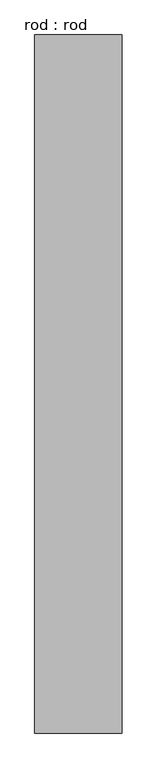
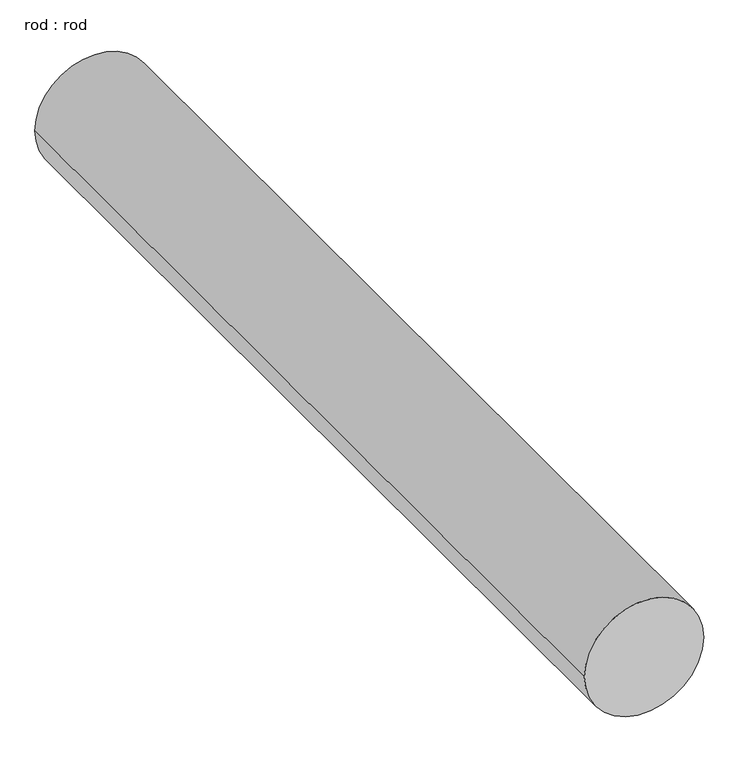
"""IFC4 building model written with IfcOpenShell, lengths in millimetres: proxy geometry, rod : rod."""

from ifc_helpers import new_model, si_unit, point, frame, frame_2d, origin, place, context, project, spatial, circle_curve, trimmed, segment, composite_curve, outline, extrude, source, transform, mapped, element, save


def rod_rod_74fe4f4c(model_context):
    return source(origin(), model_context, "Body", "SweptSolid", [
        extrude(outline(composite_curve([segment(trimmed(circle_curve(frame_2d((0.0108462, 0.0)), 200.0), [point((0.0108462, 200.0))], [point((0.0108462, -200.0))], False, "CARTESIAN"), True, "CONTINUOUS"), segment(trimmed(circle_curve(frame_2d((0.0108462, 0.0)), 200.0), [point((0.0108462, -200.0))], [point((0.0108462, 200.0))], False, "CARTESIAN"), True, "CONTINUOUS")], self_intersect=False)), frame((0.0, 2496.3000439, 0.0), z_axis=(0.0, 1.0, 0.0), x_axis=(0.0, 0.0, 1.0)), (0.0, 0.0, 1.0), 3192.8571429),
    ])


if __name__ == "__main__":
    model = new_model("IFC4")
    model_context = context("Model", 3, world=origin())
    ifc_project = project(units=[si_unit("LENGTHUNIT", "METRE", prefix="MILLI")], contexts=[model_context])
    site = spatial("IfcSite", under=ifc_project)
    building = spatial("IfcBuilding", under=site)
    placement = place(None, origin())
    rod_rod_shape = rod_rod_74fe4f4c(model_context)
    element("IfcBuildingElementProxy", 1, Name="rod : rod", ObjectType="rod : rod", at=placement, inside=building, context=model_context, shape_type="MappedRepresentation", body=[
        mapped(rod_rod_shape, transform((0.0, 0.0, 0.0), x_axis=(1.0, 0.0, 0.0), y_axis=(0.0, 1.0, 0.0), z_axis=(0.0, 0.0, 1.0))),
    ])
    save(model, "model.ifc")

# Revit data of these elements
# Type "rod : rod"
#   Default Elevation = 0
